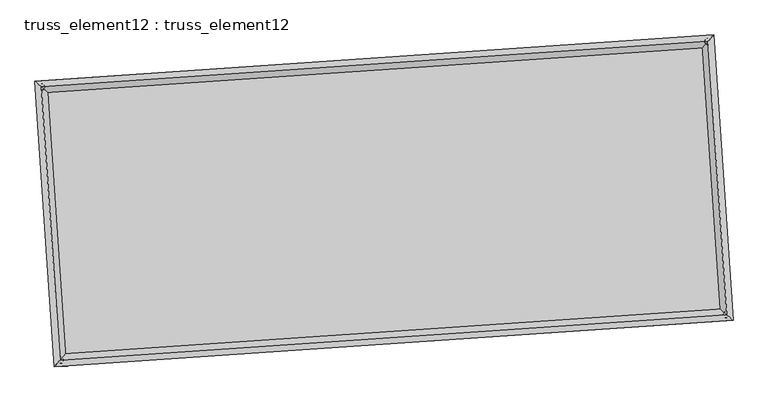
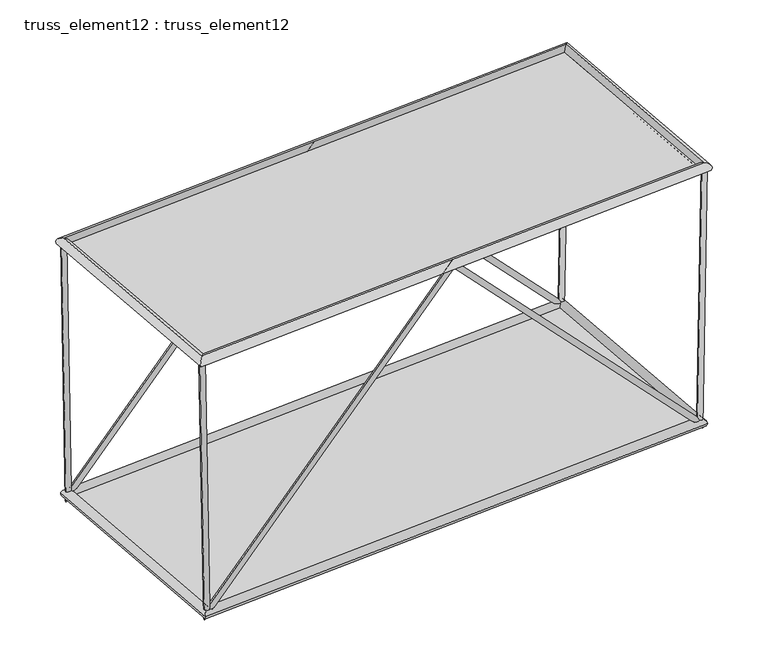
"""IFC4 building model written with IfcOpenShell, lengths in millimetres: plate geometry, truss_element12 : truss_element12."""

import ifcopenshell
import ifcopenshell.guid

model = None  # the IFC model being written
_history = None  # IfcOwnerHistory: only IFC2X3 demands one
_inside = {}  # id of a spatial element -> (the spatial element, [elements in it])
_under = {}  # id of a project, library or spatial element -> (it, [spatial elements below it])
_declared = {}  # id of a project -> (the project, [libraries it declares])
_typed = {}  # id of a type object -> (the type object, [elements of that type])
_made_of = {}  # id of a material, layer set ... -> (it, [elements and type objects made of it])


def new_model(schema):
    """Start an empty IFC model of exactly this schema.

    Asked for "IFC4X3", IfcOpenShell would pick the latest addendum, in which some entities
    have other attributes; the version numbers below select the first issue.
    IFC2X3 requires an IfcOwnerHistory on every rooted entity: one is made here for all.
    """
    global model, _history
    if schema == "IFC4X3":
        model = ifcopenshell.file(schema_version=(4, 3, 0, 0))
    else:
        model = ifcopenshell.file(schema=schema)
    _inside.clear()
    _under.clear()
    _declared.clear()
    _typed.clear()
    _made_of.clear()
    _history = None
    if model.schema == "IFC2X3":
        org = make("IfcOrganization", Name="unknown")
        user = make(
            "IfcPersonAndOrganization",
            ThePerson=make("IfcPerson", FamilyName="unknown"),
            TheOrganization=org,
        )
        app = make(
            "IfcApplication",
            ApplicationDeveloper=org,
            Version="unknown",
            ApplicationFullName="unknown",
            ApplicationIdentifier="unknown",
        )
        _history = make(
            "IfcOwnerHistory",
            OwningUser=user,
            OwningApplication=app,
            ChangeAction="ADDED",
            CreationDate=0,
        )
    return model


def make(cls, **values):
    """One entity of the class cls with the attributes given. An attribute that is None is left unset."""
    return model.create_entity(
        cls, **{name: value for name, value in values.items() if value is not None}
    )


def rooted(cls, **values):
    """An entity with a GlobalId (a new one), such as an element, a storey or a relation."""
    return make(cls, GlobalId=ifcopenshell.guid.new(), OwnerHistory=_history, **values)


def si_unit(unit_type, name, prefix=None):
    """IfcSIUnit, for example si_unit("LENGTHUNIT", "METRE", prefix="MILLI")."""
    return make("IfcSIUnit", UnitType=unit_type, Prefix=prefix, Name=name)


def assignment(units):
    """IfcUnitAssignment: the units of a project."""
    return None if units is None else make("IfcUnitAssignment", Units=units)


def point(xyz):
    """IfcCartesianPoint."""
    return None if xyz is None else make("IfcCartesianPoint", Coordinates=xyz)


def direction(xyz):
    """IfcDirection."""
    return None if xyz is None else make("IfcDirection", DirectionRatios=xyz)


def frame(location, z_axis=None, x_axis=None):
    """IfcAxis2Placement3D, a coordinate frame: its origin and axes. An axis left out is left unset."""
    return make(
        "IfcAxis2Placement3D",
        Location=point(location),
        Axis=direction(z_axis),
        RefDirection=direction(x_axis),
    )


def origin():
    """The frame at (0, 0, 0) with its axes left unset."""
    return frame((0.0, 0.0, 0.0))


def origin_with_axes():
    """The frame at (0, 0, 0) with the z axis (0, 0, 1) and the x axis (1, 0, 0) written out."""
    return frame((0.0, 0.0, 0.0), z_axis=(0.0, 0.0, 1.0), x_axis=(1.0, 0.0, 0.0))


def place(relative_to, where):
    """IfcLocalPlacement: puts the frame where relative to a parent placement (None: the world)."""
    return make(
        "IfcLocalPlacement", PlacementRelTo=relative_to, RelativePlacement=where
    )


def context(
    kind, dimensions, precision=None, world=None, true_north=None, identifier=None
):
    """IfcGeometricRepresentationContext, for example the 3D "Model" context."""
    return make(
        "IfcGeometricRepresentationContext",
        ContextIdentifier=identifier,
        ContextType=kind,
        CoordinateSpaceDimension=dimensions,
        Precision=precision,
        WorldCoordinateSystem=world,
        TrueNorth=true_north,
    )


def project(units=None, contexts=None):
    """IfcProject with its units and contexts."""
    return rooted(
        "IfcProject",
        Name="project",
        RepresentationContexts=contexts,
        UnitsInContext=assignment(units),
    )


def spatial(cls, under=None, at=None, **own):
    """A site, building, storey or space (cls), placed at a placement, below another one or the project."""
    s = rooted(cls, ObjectPlacement=at, **own)
    if under is not None:
        _under.setdefault(under.id(), (under, []))[1].append(s)
    return s


def polyline(points):
    """IfcPolyline through the points."""
    return make("IfcPolyline", Points=[point(p) for p in points])


def circle_curve(where, radius):
    """IfcCircle in the frame where."""
    return make("IfcCircle", Position=where, Radius=radius)


def ellipse_curve(where, semi_axis1, semi_axis2):
    """IfcEllipse in the frame where."""
    return make(
        "IfcEllipse", Position=where, SemiAxis1=semi_axis1, SemiAxis2=semi_axis2
    )


def outline(outer, holes=None, kind="AREA"):
    """IfcArbitraryClosedProfileDef: a profile drawn as a closed curve; with holes, ...WithVoids."""
    if holes is None:
        return make("IfcArbitraryClosedProfileDef", ProfileType=kind, OuterCurve=outer)
    return make(
        "IfcArbitraryProfileDefWithVoids",
        ProfileType=kind,
        OuterCurve=outer,
        InnerCurves=holes,
    )


def extrude(swept, where, along, depth):
    """IfcExtrudedAreaSolid: the profile swept, set in the frame where, extruded along a direction by depth."""
    return make(
        "IfcExtrudedAreaSolid",
        SweptArea=swept,
        Position=where,
        ExtrudedDirection=direction(along),
        Depth=depth,
    )


def shape(context_of_items, identifier, shape_type, items):
    """IfcShapeRepresentation: the items that make up one representation, for example the "Body"."""
    return make(
        "IfcShapeRepresentation",
        ContextOfItems=context_of_items,
        RepresentationIdentifier=identifier,
        RepresentationType=shape_type,
        Items=items,
    )


def source(mapping_origin, context_of_items, identifier, shape_type, items):
    """IfcRepresentationMap: a shape defined once, which mapped items show again and again."""
    return make(
        "IfcRepresentationMap",
        MappingOrigin=mapping_origin,
        MappedRepresentation=shape(context_of_items, identifier, shape_type, items),
    )


def transform(
    local_origin,
    x_axis=None,
    y_axis=None,
    z_axis=None,
    scale=None,
    scale2=None,
    scale3=None,
    uniform=True,
):
    """IfcCartesianTransformationOperator3D, or its non-uniform kind. x_axis, y_axis, z_axis: its Axis1, 2, 3."""
    if uniform:
        return make(
            "IfcCartesianTransformationOperator3D",
            Axis1=direction(x_axis),
            Axis2=direction(y_axis),
            LocalOrigin=point(local_origin),
            Scale=scale,
            Axis3=direction(z_axis),
        )
    return make(
        "IfcCartesianTransformationOperator3DnonUniform",
        Axis1=direction(x_axis),
        Axis2=direction(y_axis),
        LocalOrigin=point(local_origin),
        Scale=scale,
        Axis3=direction(z_axis),
        Scale2=scale2,
        Scale3=scale3,
    )


def mapped(mapping_source, mapping_target):
    """IfcMappedItem: shows the shape of a source again, moved by a transform."""
    return make(
        "IfcMappedItem", MappingSource=mapping_source, MappingTarget=mapping_target
    )


def made_of(thing, what):
    """Note that an element or type object is made of a material, layer set ...; save() writes the relation."""
    if what is not None:
        _made_of.setdefault(what.id(), (what, []))[1].append(thing)
    return thing


def element(
    cls,
    number,
    at=None,
    inside=None,
    cuts=None,
    type_object=None,
    material=None,
    context=None,
    identifier="Body",
    shape_type=None,
    held_by="IfcProductDefinitionShape",
    body=None,
    shapes=None,
    **own,
):
    """One element of the class cls, such as IfcWall. Its Tag is "e" and its number.

    at: its placement. inside: the storey or other place that contains it. cuts: it is an
    opening in that element (IfcRelVoidsElement). A single representation is given by context,
    identifier, shape_type and body (its items); several are given by shapes. held_by: the class
    of the entity that holds the representations. save() writes the other relations.
    """
    e = rooted(cls, Tag="e%d" % number, ObjectPlacement=at, **own)
    if body is not None:
        shapes = [shape(context, identifier, shape_type, body)]
    if shapes is not None:
        e.Representation = make(held_by, Representations=shapes)
    if inside is not None:
        _inside.setdefault(inside.id(), (inside, []))[1].append(e)
    if cuts is not None:
        rooted(
            "IfcRelVoidsElement", RelatingBuildingElement=cuts, RelatedOpeningElement=e
        )
    if type_object is not None:
        _typed.setdefault(type_object.id(), (type_object, []))[1].append(e)
    return made_of(e, material)


def aggregate(whole, parts):
    """IfcRelAggregates: a whole, such as a stair, and the parts it consists of."""
    return rooted("IfcRelAggregates", RelatingObject=whole, RelatedObjects=parts)


def save(model, path):
    """Write the relations noted so far, then the file.

    IfcRelAggregates (storeys below a building ...), IfcRelContainedInSpatialStructure (elements
    in a storey), IfcRelDefinesByType, IfcRelAssociatesMaterial and IfcRelDeclares: one each for
    every whole, place, type object, material and project.
    """
    for whole, parts in _under.values():
        aggregate(whole, parts)
    for where, things in _inside.values():
        rooted(
            "IfcRelContainedInSpatialStructure",
            RelatedElements=things,
            RelatingStructure=where,
        )
    for kind, things in _typed.values():
        rooted("IfcRelDefinesByType", RelatedObjects=things, RelatingType=kind)
    for what, things in _made_of.values():
        rooted("IfcRelAssociatesMaterial", RelatedObjects=things, RelatingMaterial=what)
    for by, libraries in _declared.values():
        rooted("IfcRelDeclares", RelatingContext=by, RelatedDefinitions=libraries)
    model.write(path)


def plane_surface(at):
    """IfcPlane: the flat surface through the origin of the frame at, square to its z axis."""
    return make("IfcPlane", Position=at)


def cylinder_surface(at, radius):
    """IfcCylindricalSurface: all points at the distance radius from the z axis of the frame at."""
    return make("IfcCylindricalSurface", Position=at, Radius=radius)


def advanced_brep(points, edges, surfaces, faces):
    """IfcAdvancedBrep: a solid bounded by faces that lie on surfaces and meet in shared edges.

    An edge is (start, end): straight between two places in points (the first is 0);
    or (start, end, curve); or (start, end, curve, False) where it runs against its curve.
    A face is (place in surfaces, loops), or (place, loops, False) where it looks against
    its surface's normal. A loop lists edges by number (the first is 1), with a minus sign
    where the edge is run from its end to its start. The first loop is the outer one.
    """
    corners = [point(p) for p in points]
    vertices = [make("IfcVertexPoint", VertexGeometry=c) for c in corners]
    made = []
    for start, end, *more in edges:
        made.append(
            make(
                "IfcEdgeCurve",
                EdgeStart=vertices[start],
                EdgeEnd=vertices[end],
                EdgeGeometry=more[0] if more else make("IfcPolyline", Points=[corners[start], corners[end]]),
                SameSense=more[1] if len(more) > 1 else True,
            )
        )
    hull = []
    for where, loops, *sense in faces:
        bounds = []
        for j, loop in enumerate(loops):
            ring = [make("IfcOrientedEdge", EdgeElement=made[abs(k) - 1], Orientation=k > 0) for k in loop]
            bounds.append(
                make(
                    "IfcFaceOuterBound" if j == 0 else "IfcFaceBound",
                    Bound=make("IfcEdgeLoop", EdgeList=ring),
                    Orientation=True,
                )
            )
        hull.append(make("IfcAdvancedFace", Bounds=bounds, FaceSurface=surfaces[where], SameSense=sense[0] if sense else True))
    return make("IfcAdvancedBrep", Outer=make("IfcClosedShell", CfsFaces=hull))


def truss_element12_truss_element12_ae3a266e(model_context):
    return source(origin(), model_context, "Body", "SolidModel", [
        advanced_brep(
        [(-3756.1802311, 2270.0027691, 5000.0761995), (-3855.2669443, 2256.6426372, 4998.2513335), (-3667.1577697, 2276.0728724, 121.8875578), (-3761.8291131, 2263.0138077, -121.8875578), (1063.0031207, 2598.6045625, 5071.2944622), (1063.4620192, 2592.0320674, 4927.0589367), (5794.562368, 2921.2316012, 121.8973846), (5890.198609, 2921.1488873, -121.8973846), (5882.1969104, 2927.2070675, 5000.0878443), (5982.180545, 2927.4207859, 4998.2914205)],
        [
            (0, 1, circle_curve(frame((-3805.7235877, 2263.3227032, 4999.1637665), z_axis=(-0.01824602926340183, -0.0012441273758235993, 0.9998327532958659), x_axis=(-0.13360167870548645, 0.9910343786135793, -0.0012049286588313372)), 50.0)),
            (1, 0, circle_curve(frame((-3805.7235877, 2263.3227032, 4999.1637665), z_axis=(-0.01824602926340183, -0.0012441273758235993, 0.9998327532958659), x_axis=(-0.13360167870548645, 0.9910343786135793, -0.0012049286588313372)), 50.0)),
            (0, 2),
            (2, 3, ellipse_curve(frame((-3714.4934414, 2269.54334, 0.0), z_axis=(-0.9291499210086428, -0.06335520108406499, 0.3642341867332479), x_axis=(0.3633904003865977, 0.024778210026124285, 0.93130739136698)), 131.1628889, 50.0)),
            (3, 1),
            (3, 2, ellipse_curve(frame((-3714.4934414, 2269.54334, 0.0), z_axis=(-0.9291499210086428, -0.06335520108406499, 0.3642341867332479), x_axis=(0.3633904003865977, 0.024778210026124285, 0.93130739136698)), 131.1628889, 50.0)),
            (2, 4),
            (4, 5, ellipse_curve(frame((1063.23257, 2595.3183149, 4999.1766994), z_axis=(-0.9976833933192731, -0.06802823804080799, -7.432364115787789e-05), x_axis=(7.415146271864652e-05, 5.056106369626309e-06, -0.9999999972379982)), 72.2747993, 50.0)),
            (5, 3),
            (5, 4, ellipse_curve(frame((1063.23257, 2595.3183149, 4999.1766994), z_axis=(-0.9976833933192731, -0.06802823804080799, -7.432364115787789e-05), x_axis=(7.415146271864652e-05, 5.056106369626309e-06, -0.9999999972379982)), 72.2747993, 50.0)),
            (4, 6),
            (6, 7, ellipse_curve(frame((5842.3804885, 2921.1902443, 0.0), z_axis=(-0.9290710914132949, -0.06334982599361544, -0.36443614892966847), x_axis=(-0.36359189471660097, -0.02479194915854102, 0.9312283787306489)), 131.1845933, 50.0)),
            (7, 5),
            (7, 6, ellipse_curve(frame((5842.3804885, 2921.1902443, 0.0), z_axis=(-0.9290710914132949, -0.06334982599361544, -0.36443614892966847), x_axis=(-0.36359189471660097, -0.02479194915854102, 0.9312283787306489)), 131.1845933, 50.0)),
            (8, 9, circle_curve(frame((5932.1887277, 2927.3139267, 4999.1896324), z_axis=(0.01796164783284282, 0.0012247364871029384, 0.9998379264799202), x_axis=(-0.0021588384546528737, 0.99999696622927, -0.0011861487187809492)), 50.0)),
            (9, 8, circle_curve(frame((5932.1887277, 2927.3139267, 4999.1896324), z_axis=(0.01796164783284282, 0.0012247364871029384, 0.9998379264799202), x_axis=(-0.0021588384546528737, 0.99999696622927, -0.0011861487187809492)), 50.0)),
            (6, 8),
            (9, 7),
        ],
        [
            plane_surface(frame((-3805.7235877, 2313.3226645, 4999.2259832), z_axis=(-0.018246029263402925, -0.0012441273758274742, 0.999832753295866), x_axis=(0.9998335273514882, -2.270416412919475e-05, 0.01824601513760983))),
            cylinder_surface(frame((-3805.7235877, 2263.3227032, 4999.1637665), z_axis=(-0.018246029263401832, -0.0012441273758235995, 0.9998327532958661), x_axis=(-0.13360167870548645, 0.9910343786135793, -0.0012049286588313372)), 50.0),
            cylinder_surface(frame((-3714.4934414, 2269.54334, 0.0), z_axis=(-0.6901478836925812, -0.04705856069127947, -0.7221366840843337), x_axis=(-0.02041276416893784, 0.9987523004244808, -0.045575886780083084)), 50.0),
            cylinder_surface(frame((1063.23257, 2595.3183149, 4999.1766994), z_axis=(-0.6902549710503421, -0.04706586257113229, 0.7220338492901334), x_axis=(-0.11534133347445269, 0.992279482140813, -0.04558295859962826)), 50.0),
            plane_surface(frame((5932.1887277, 2877.3139642, 4999.2508791), z_axis=(0.017961647832841293, 0.001224736487099467, 0.9998379264799202), x_axis=(0.9998386765909434, -2.2001834880214226e-05, -0.017961634357437358))),
            cylinder_surface(frame((5842.3804885, 2921.1902443, 0.0), z_axis=(-0.01796164783284282, -0.0012247364871029384, -0.9998379264799202), x_axis=(-0.0021588384546528737, 0.99999696622927, -0.0011861487187809492)), 50.0),
        ],
        [
            (0, [[1, 2]]),
            (1, [[-1, 3, 4, 5]]),
            (1, [[-2, -5, 6, -3]]),
            (2, [[-4, 7, 8, 9]]),
            (2, [[-6, -9, 10, -7]]),
            (3, [[-8, 11, 12, 13]]),
            (3, [[-10, -13, 14, -11]]),
            (4, [[15, 16]]),
            (5, [[-12, 17, -16, 18]]),
            (5, [[-14, -18, -15, -17]]),
        ],
    ),
        advanced_brep(
        [(-3484.0672782, -1720.7308152, 5000.0761995), (-3583.1539914, -1734.0909471, 4998.2513335), (-3395.0448168, -1714.6607119, 121.8875578), (-3489.7161602, -1727.7197766, -121.8875578), (1335.1160737, -1392.1290218, 5071.2944622), (1335.5749721, -1398.7015169, 4927.0589367), (6066.6753209, -1069.5019831, 121.8973846), (6162.3115619, -1069.584697, -121.8973846), (6154.3098633, -1063.5265168, 5000.0878443), (6254.2934979, -1063.3127984, 4998.2914205)],
        [
            (0, 1, circle_curve(frame((-3533.6106348, -1727.4108811, 4999.1637665), z_axis=(-0.01824602926340309, -0.0012441273758237222, 0.9998327532958659), x_axis=(-0.1336016787054862, 0.9910343786135793, -0.0012049286588313795)), 50.0)),
            (1, 0, circle_curve(frame((-3533.6106348, -1727.4108811, 4999.1637665), z_axis=(-0.01824602926340309, -0.0012441273758237222, 0.9998327532958659), x_axis=(-0.1336016787054862, 0.9910343786135793, -0.0012049286588313795)), 50.0)),
            (0, 2),
            (2, 3, ellipse_curve(frame((-3442.3804885, -1721.1902443, 0.0), z_axis=(-0.9291499210086432, -0.06335520108406512, 0.364234186733247), x_axis=(0.3633904003865968, 0.024778210026124223, 0.9313073913669805)), 131.1628889, 50.0)),
            (3, 1),
            (3, 2, ellipse_curve(frame((-3442.3804885, -1721.1902443, 0.0), z_axis=(-0.9291499210086432, -0.06335520108406512, 0.364234186733247), x_axis=(0.3633904003865968, 0.024778210026124223, 0.9313073913669805)), 131.1628889, 50.0)),
            (2, 4),
            (4, 5, ellipse_curve(frame((1335.3455229, -1395.4152694, 4999.1766994), z_axis=(-0.9976833933192731, -0.06802823804080792, -7.432364116044547e-05), x_axis=(7.415146272126043e-05, 5.0561063696839735e-06, -0.999999997237998)), 72.2747993, 50.0)),
            (5, 3),
            (5, 4, ellipse_curve(frame((1335.3455229, -1395.4152694, 4999.1766994), z_axis=(-0.9976833933192731, -0.06802823804080792, -7.432364116044547e-05), x_axis=(7.415146272126043e-05, 5.0561063696839735e-06, -0.999999997237998)), 72.2747993, 50.0)),
            (4, 6),
            (6, 7, ellipse_curve(frame((6114.4934414, -1069.54334, 0.0), z_axis=(-0.9290710914132941, -0.06334982599361536, -0.3644361489296707), x_axis=(-0.363591894716603, -0.024791949158541025, 0.9312283787306479)), 131.1845933, 50.0)),
            (7, 5),
            (7, 6, ellipse_curve(frame((6114.4934414, -1069.54334, 0.0), z_axis=(-0.9290710914132941, -0.06334982599361536, -0.3644361489296707), x_axis=(-0.363591894716603, -0.024791949158541025, 0.9312283787306479)), 131.1845933, 50.0)),
            (8, 9, circle_curve(frame((6204.3016806, -1063.4196576, 4999.1896324), z_axis=(0.01796164783284177, 0.0012247364871029872, 0.9998379264799201), x_axis=(-0.0021588384546530333, 0.99999696622927, -0.0011861487187809978)), 50.0)),
            (9, 8, circle_curve(frame((6204.3016806, -1063.4196576, 4999.1896324), z_axis=(0.01796164783284177, 0.0012247364871029872, 0.9998379264799201), x_axis=(-0.0021588384546530333, 0.99999696622927, -0.0011861487187809978)), 50.0)),
            (6, 8),
            (9, 7),
        ],
        [
            plane_surface(frame((-3533.6106348, -1677.4109198, 4999.2259832), z_axis=(-0.018246029263402925, -0.0012441273758274944, 0.999832753295866), x_axis=(0.9998335273514882, -2.270416412919475e-05, 0.01824601513760983))),
            cylinder_surface(frame((-3533.6106348, -1727.4108811, 4999.1637665), z_axis=(-0.018246029263403095, -0.0012441273758237224, 0.9998327532958661), x_axis=(-0.1336016787054862, 0.9910343786135793, -0.0012049286588313795)), 50.0),
            cylinder_surface(frame((-3442.3804885, -1721.1902443, 0.0), z_axis=(-0.6901478836925803, -0.04705856069127945, -0.7221366840843344), x_axis=(-0.02041276416893806, 0.9987523004244808, -0.045575886780082814)), 50.0),
            cylinder_surface(frame((1335.3455229, -1395.4152694, 4999.1766994), z_axis=(-0.690254971050345, -0.04706586257113233, 0.7220338492901303), x_axis=(-0.11534133347445193, 0.992279482140813, -0.04558295859962813)), 50.0),
            plane_surface(frame((6204.3016806, -1113.4196201, 4999.2508791), z_axis=(0.017961647832841293, 0.001224736487099487, 0.9998379264799202), x_axis=(0.9998386765909434, -2.2001834880214226e-05, -0.017961634357437358))),
            cylinder_surface(frame((6114.4934414, -1069.54334, 0.0), z_axis=(-0.017961647832841772, -0.0012247364871029874, -0.9998379264799203), x_axis=(-0.0021588384546530333, 0.99999696622927, -0.0011861487187809978)), 50.0),
        ],
        [
            (0, [[1, 2]]),
            (1, [[-1, 3, 4, 5]]),
            (1, [[-2, -5, 6, -3]]),
            (2, [[-4, 7, 8, 9]]),
            (2, [[-6, -9, 10, -7]]),
            (3, [[-8, 11, 12, 13]]),
            (3, [[-10, -13, 14, -11]]),
            (4, [[15, 16]]),
            (5, [[-12, 17, -16, 18]]),
            (5, [[-14, -18, -15, -17]]),
        ],
    ),
        advanced_brep(
        [(-3533.6038857, -1727.4034009, 4909.1637668), (-3533.6173839, -1727.4183614, 5089.1637662), (-3805.7312897, 2263.3291981, 5089.1637662), (-3805.7158857, 2263.3162083, 4909.1637668), (5932.1950008, 2927.3213745, 5089.1896321), (5932.1824545, 2927.3064789, 4909.1896327), (6204.3089067, -1063.426185, 5089.1896321), (6204.2944545, -1063.4131303, 4909.1896327)],
        [
            (0, 1, ellipse_curve(frame((-3533.6106348, -1727.4108811, 4999.1637665), z_axis=(-0.7535719234029822, 0.6573654662782481, -1.8738715656892282e-06), x_axis=(-0.657365466275602, -0.7535719234052904, -1.8738715718147318e-06)), 127.2792206, 90.0)),
            (1, 2),
            (2, 3, ellipse_curve(frame((-3805.7235877, 2263.3227032, 4999.1637665), z_axis=(-0.657365466275602, -0.7535719234052904, -1.873871569304263e-06), x_axis=(0.7535719234029821, -0.6573654662782482, 1.8738715631787596e-06)), 127.2792206, 90.0)),
            (3, 0),
            (1, 0, ellipse_curve(frame((-3533.6106348, -1727.4108811, 4999.1637665), z_axis=(-0.7535719234029822, 0.6573654662782481, -1.8738715656892282e-06), x_axis=(-0.657365466275602, -0.7535719234052904, -1.8738715718147318e-06)), 127.2792206, 90.0)),
            (3, 2, ellipse_curve(frame((-3805.7235877, 2263.3227032, 4999.1637665), z_axis=(-0.657365466275602, -0.7535719234052904, -1.873871569304263e-06), x_axis=(0.7535719234029821, -0.6573654662782482, 1.8738715631787596e-06)), 127.2792206, 90.0)),
            (2, 4),
            (4, 5, ellipse_curve(frame((5932.1887277, 2927.3139267, 4999.1896324), z_axis=(-0.7535719234029844, 0.6573654662782455, -1.873871569304268e-06), x_axis=(-0.6573654662755994, -0.7535719234052927, -1.8738715631787545e-06)), 127.2792206, 90.0)),
            (5, 3),
            (5, 4, ellipse_curve(frame((5932.1887277, 2927.3139267, 4999.1896324), z_axis=(-0.7535719234029844, 0.6573654662782455, -1.873871569304268e-06), x_axis=(-0.6573654662755994, -0.7535719234052927, -1.8738715631787545e-06)), 127.2792206, 90.0)),
            (4, 6),
            (6, 7, ellipse_curve(frame((6204.3016806, -1063.4196576, 4999.1896324), z_axis=(0.6573654662755994, 0.7535719234052927, 1.8738715656892233e-06), x_axis=(-0.7535719234029844, 0.6573654662782457, -1.8738715718147367e-06)), 127.2792206, 90.0)),
            (7, 5),
            (7, 6, ellipse_curve(frame((6204.3016806, -1063.4196576, 4999.1896324), z_axis=(0.6573654662755994, 0.7535719234052927, 1.8738715656892233e-06), x_axis=(-0.7535719234029844, 0.6573654662782457, -1.8738715718147367e-06)), 127.2792206, 90.0)),
            (6, 1),
            (0, 7),
        ],
        [
            cylinder_surface(frame((-3533.6106348, -1727.4108811, 4999.1637665), z_axis=(0.06802823822870267, -0.9976833960748765, 0.0), x_axis=(-0.9976833928446474, -0.06802823800844562, -8.047023891255004e-05)), 90.0),
            cylinder_surface(frame((-3805.7235877, 2263.3227032, 4999.1637665), z_axis=(-0.9976833960713732, -0.0680282382284653, -2.6500545831240593e-06), x_axis=(-0.0680282378169653, 0.9976833930679299, -7.78201843331188e-05)), 90.0),
            cylinder_surface(frame((5932.1887277, 2927.3139267, 4999.1896324), z_axis=(-0.06802823822870929, 0.9976833960748762, 0.0), x_axis=(0.997683393256147, 0.06802823803651087, -7.517012975368756e-05)), 90.0),
            cylinder_surface(frame((6204.3016806, -1063.4196576, 4999.1896324), z_axis=(0.9976833960713731, 0.06802823822846524, 2.6500545866743975e-06), x_axis=(0.06802823822846522, -0.9976833930398712, -7.782018432800606e-05)), 90.0),
        ],
        [
            (0, [[1, 2, 3, 4]]),
            (0, [[5, -4, 6, -2]]),
            (1, [[-3, 7, 8, 9]]),
            (1, [[-6, -9, 10, -7]]),
            (2, [[-8, 11, 12, 13]]),
            (2, [[-10, -13, 14, -11]]),
            (3, [[-12, 15, -1, 16]]),
            (3, [[-14, -16, -5, -15]]),
        ],
    ),
        advanced_brep(
        [(-3358.7115243, -1625.2761972, 0.0), (-3526.0494527, -1817.1042913, 0.0), (-3810.4074885, 2353.2123043, 0.0), (-3618.5793943, 2185.8743758, 0.0), (5926.0494527, 3017.1042913, 0.0), (5758.7115243, 2825.2761972, 0.0), (6210.4074885, -1153.2123043, 0.0), (6018.5793943, -985.8743758, 0.0)],
        [
            (0, 1, ellipse_curve(frame((-3442.3804885, -1721.1902443, 0.0), z_axis=(-0.7535719234054582, 0.6573654662780805, 0.0), x_axis=(-0.6573654662780805, -0.7535719234054583, 0.0)), 127.2792206, 90.0)),
            (1, 2),
            (2, 3, ellipse_curve(frame((-3714.4934414, 2269.54334, 0.0), z_axis=(-0.6573654662780805, -0.7535719234054583, 0.0), x_axis=(0.7535719234054583, -0.6573654662780803, 0.0)), 127.2792206, 90.0)),
            (3, 0),
            (1, 0, ellipse_curve(frame((-3442.3804885, -1721.1902443, 0.0), z_axis=(-0.7535719234054582, 0.6573654662780805, 0.0), x_axis=(-0.6573654662780805, -0.7535719234054583, 0.0)), 127.2792206, 90.0)),
            (3, 2, ellipse_curve(frame((-3714.4934414, 2269.54334, 0.0), z_axis=(-0.6573654662780805, -0.7535719234054583, 0.0), x_axis=(0.7535719234054583, -0.6573654662780803, 0.0)), 127.2792206, 90.0)),
            (2, 4),
            (4, 5, ellipse_curve(frame((5842.3804885, 2921.1902443, 0.0), z_axis=(-0.7535719234054603, 0.657365466278078, 0.0), x_axis=(-0.6573654662780781, -0.7535719234054603, 0.0)), 127.2792206, 90.0)),
            (5, 3),
            (5, 4, ellipse_curve(frame((5842.3804885, 2921.1902443, 0.0), z_axis=(-0.7535719234054603, 0.657365466278078, 0.0), x_axis=(-0.6573654662780781, -0.7535719234054603, 0.0)), 127.2792206, 90.0)),
            (4, 6),
            (6, 7, ellipse_curve(frame((6114.4934414, -1069.54334, 0.0), z_axis=(0.6573654662780782, 0.7535719234054603, 0.0), x_axis=(-0.7535719234054604, 0.657365466278078, 0.0)), 127.2792206, 90.0)),
            (7, 5),
            (7, 6, ellipse_curve(frame((6114.4934414, -1069.54334, 0.0), z_axis=(0.6573654662780782, 0.7535719234054603, 0.0), x_axis=(-0.7535719234054604, 0.657365466278078, 0.0)), 127.2792206, 90.0)),
            (6, 1),
            (0, 7),
        ],
        [
            cylinder_surface(frame((-3442.3804885, -1721.1902443, 0.0), z_axis=(0.0680282382287011, -0.9976833960748767, 0.0), x_axis=(-0.9976833960748767, -0.0680282382287011, 0.0)), 90.0),
            cylinder_surface(frame((-3714.4934414, 2269.54334, 0.0), z_axis=(-0.9976833960748765, -0.06802823822870233, 0.0), x_axis=(-0.06802823822870233, 0.9976833960748765, 0.0)), 90.0),
            cylinder_surface(frame((5842.3804885, 2921.1902443, 0.0), z_axis=(-0.0680282382287075, 0.9976833960748761, 0.0), x_axis=(0.9976833960748761, 0.0680282382287075, 0.0)), 90.0),
            cylinder_surface(frame((6114.4934414, -1069.54334, 0.0), z_axis=(0.9976833960748767, 0.06802823822870217, 0.0), x_axis=(0.06802823822870217, -0.9976833960748767, 0.0)), 90.0),
        ],
        [
            (0, [[1, 2, 3, 4]]),
            (0, [[5, -4, 6, -2]]),
            (1, [[-3, 7, 8, 9]]),
            (1, [[-6, -9, 10, -7]]),
            (2, [[-8, 11, 12, 13]]),
            (2, [[-10, -13, 14, -11]]),
            (3, [[-12, 15, -1, 16]]),
            (3, [[-14, -16, -5, -15]]),
        ],
    ),
        extrude(outline(polyline([(-3442.3804885, -1721.1902443), (-3714.4934414, 2269.54334), (5842.3804885, 2921.1902443), (6114.4934414, -1069.54334), (-3442.3804885, -1721.1902443)])), origin_with_axes(), (0.0, 0.0, 1.0), 20.0),
        extrude(outline(polyline([(-2000.0, 4880.2617913), (2000.0, 4880.2617913), (2000.0, -4880.2617914), (-2000.0, -4880.2617914), (-2000.0, 4880.2617913)])), frame((1199.2890464, 599.9515228, 4999.1766994), z_axis=(-2.643915455980416e-06, -1.802785488212624e-07, 0.9999999999964887), x_axis=(-0.06802823822870048, 0.9976833960748767, 0.0)), (0.0, 0.0, 1.0), 20.0),
    ])


if __name__ == "__main__":
    model = new_model("IFC4")
    model_context = context("Model", 3, world=origin())
    ifc_project = project(units=[si_unit("LENGTHUNIT", "METRE", prefix="MILLI")], contexts=[model_context])
    site = spatial("IfcSite", under=ifc_project)
    building = spatial("IfcBuilding", under=site)
    placement = place(None, origin())
    truss_element12_truss_element12_shape = truss_element12_truss_element12_ae3a266e(model_context)
    element("IfcPlate", 1, ObjectType="truss_element12 : truss_element12", at=placement, inside=building, context=model_context, shape_type="MappedRepresentation", body=[
        mapped(truss_element12_truss_element12_shape, transform((0.0, 0.0, 0.0), x_axis=(1.0, 0.0, 0.0), y_axis=(0.0, 1.0, 0.0), z_axis=(0.0, 0.0, 1.0))),
    ])
    save(model, "model.ifc")

# Revit data of these elements
# Type "truss_element12 : truss_element12"
#   steellbar1 = 90 mm
#   steelbar2 = 50 mm
#   offset1 = 5000 mm
#   M = Default Roof
# Element 1 (IfcPlate, "truss_element12 : truss_element12")
#   Materials on its faces: "Default Roof"
# Materials
#   "Default Roof": class "Miscellaneous", colour RGB 0 127 0, transparency 0, Comments = "Rendering appearance not upgraded Rendering appearance not upgraded ", Cost = 0
